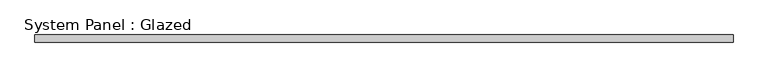
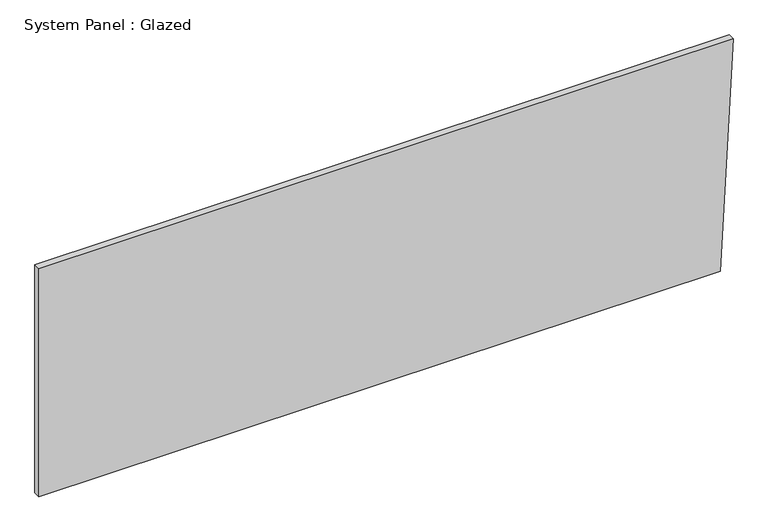
"""IFC4 building model written with IfcOpenShell, lengths in millimetres: plate geometry, System Panel : Glazed."""

from ifc_helpers import new_model, si_unit, frame, origin, place, context, project, spatial, polyline, outline, extrude, source, transform, mapped, element, save


def system_panel_glazed_a884192e(model_context):
    return source(origin(), model_context, "Body", "SweptSolid", [
        extrude(outline(polyline([(0.0, -1247.3520184), (0.0, 1202.0248119), (866.081558, 1247.3520184), (866.081558, -1247.3520184), (0.0, -1247.3520184)])), frame((0.0, -44.45, 0.0), z_axis=(0.0, 1.0, 0.0), x_axis=(0.0, 0.0, 1.0)), (0.0, 0.0, 1.0), 25.4),
    ])


if __name__ == "__main__":
    model = new_model("IFC4")
    model_context = context("Model", 3, world=origin())
    ifc_project = project(units=[si_unit("LENGTHUNIT", "METRE", prefix="MILLI")], contexts=[model_context])
    site = spatial("IfcSite", under=ifc_project)
    building = spatial("IfcBuilding", under=site)
    placement = place(None, origin())
    system_panel_glazed_shape = system_panel_glazed_a884192e(model_context)
    element("IfcPlate", 1, ObjectType="System Panel : Glazed", at=placement, inside=building, context=model_context, shape_type="MappedRepresentation", body=[
        mapped(system_panel_glazed_shape, transform((0.0, 0.0, 0.0), x_axis=(1.0, 0.0, 0.0), y_axis=(0.0, 1.0, 0.0), z_axis=(0.0, 0.0, 1.0))),
    ])
    save(model, "model.ifc")

# Revit data of these elements
# Type "System Panel : Glazed"
#   Construction Type Id = "GSP4R"
#   Analytic Construction = "1/8 in Pilkington single glazing"
#   Visual Light Transmittance = 0.9
#   Solar Heat Gain Coefficient = 0.86
#   Heat Transfer Coefficient (U) = 1.18115 BTU/(h·ft²·°F)
#   Define Thermal Properties by = 1
# Element 1 (IfcPlate, "System Panel : Glazed")
#   Materials on its faces: "Glass"
# Materials
#   "Glass": class "Glass", colour RGB 0 128 192, transparency 0.75, Description = "Soda Lime Glass", Cost = 0
